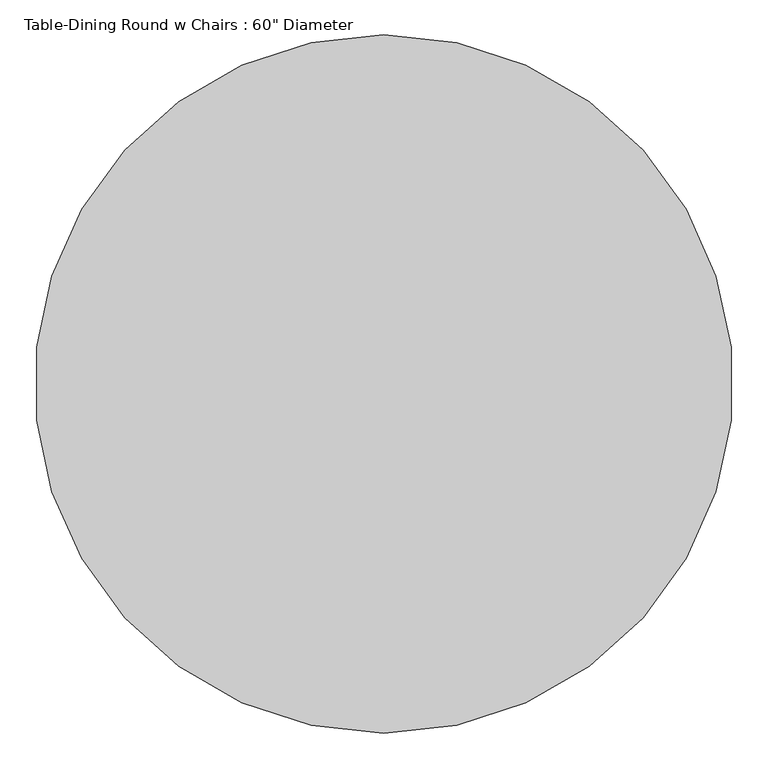
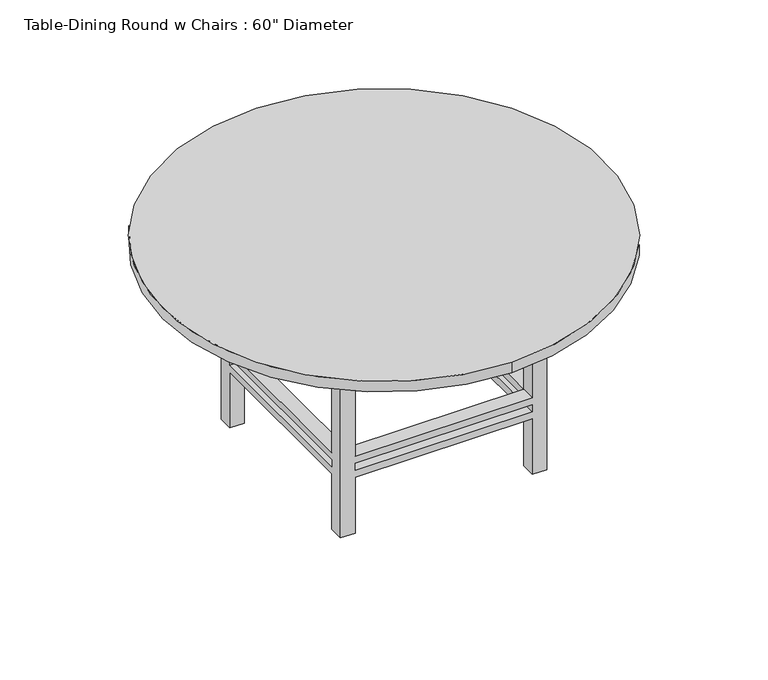
"""IFC4 building model written with IfcOpenShell, lengths in millimetres: furniture geometry."""

import ifcopenshell
import ifcopenshell.guid

model = None  # the IFC model being written
_history = None  # IfcOwnerHistory: only IFC2X3 demands one
_inside = {}  # id of a spatial element -> (the spatial element, [elements in it])
_under = {}  # id of a project, library or spatial element -> (it, [spatial elements below it])
_declared = {}  # id of a project -> (the project, [libraries it declares])
_typed = {}  # id of a type object -> (the type object, [elements of that type])
_made_of = {}  # id of a material, layer set ... -> (it, [elements and type objects made of it])


def new_model(schema):
    """Start an empty IFC model of exactly this schema.

    Asked for "IFC4X3", IfcOpenShell would pick the latest addendum, in which some entities
    have other attributes; the version numbers below select the first issue.
    IFC2X3 requires an IfcOwnerHistory on every rooted entity: one is made here for all.
    """
    global model, _history
    if schema == "IFC4X3":
        model = ifcopenshell.file(schema_version=(4, 3, 0, 0))
    else:
        model = ifcopenshell.file(schema=schema)
    _inside.clear()
    _under.clear()
    _declared.clear()
    _typed.clear()
    _made_of.clear()
    _history = None
    if model.schema == "IFC2X3":
        org = make("IfcOrganization", Name="unknown")
        user = make(
            "IfcPersonAndOrganization",
            ThePerson=make("IfcPerson", FamilyName="unknown"),
            TheOrganization=org,
        )
        app = make(
            "IfcApplication",
            ApplicationDeveloper=org,
            Version="unknown",
            ApplicationFullName="unknown",
            ApplicationIdentifier="unknown",
        )
        _history = make(
            "IfcOwnerHistory",
            OwningUser=user,
            OwningApplication=app,
            ChangeAction="ADDED",
            CreationDate=0,
        )
    return model


def make(cls, **values):
    """One entity of the class cls with the attributes given. An attribute that is None is left unset."""
    return model.create_entity(
        cls, **{name: value for name, value in values.items() if value is not None}
    )


def rooted(cls, **values):
    """An entity with a GlobalId (a new one), such as an element, a storey or a relation."""
    return make(cls, GlobalId=ifcopenshell.guid.new(), OwnerHistory=_history, **values)


def si_unit(unit_type, name, prefix=None):
    """IfcSIUnit, for example si_unit("LENGTHUNIT", "METRE", prefix="MILLI")."""
    return make("IfcSIUnit", UnitType=unit_type, Prefix=prefix, Name=name)


def assignment(units):
    """IfcUnitAssignment: the units of a project."""
    return None if units is None else make("IfcUnitAssignment", Units=units)


def point(xyz):
    """IfcCartesianPoint."""
    return None if xyz is None else make("IfcCartesianPoint", Coordinates=xyz)


def direction(xyz):
    """IfcDirection."""
    return None if xyz is None else make("IfcDirection", DirectionRatios=xyz)


def frame(location, z_axis=None, x_axis=None):
    """IfcAxis2Placement3D, a coordinate frame: its origin and axes. An axis left out is left unset."""
    return make(
        "IfcAxis2Placement3D",
        Location=point(location),
        Axis=direction(z_axis),
        RefDirection=direction(x_axis),
    )


def frame_2d(location, x_axis=None):
    """IfcAxis2Placement2D, a coordinate frame in the plane: its origin and x axis."""
    return make(
        "IfcAxis2Placement2D", Location=point(location), RefDirection=direction(x_axis)
    )


def origin():
    """The frame at (0, 0, 0) with its axes left unset."""
    return frame((0.0, 0.0, 0.0))


def place(relative_to, where):
    """IfcLocalPlacement: puts the frame where relative to a parent placement (None: the world)."""
    return make(
        "IfcLocalPlacement", PlacementRelTo=relative_to, RelativePlacement=where
    )


def context(
    kind, dimensions, precision=None, world=None, true_north=None, identifier=None
):
    """IfcGeometricRepresentationContext, for example the 3D "Model" context."""
    return make(
        "IfcGeometricRepresentationContext",
        ContextIdentifier=identifier,
        ContextType=kind,
        CoordinateSpaceDimension=dimensions,
        Precision=precision,
        WorldCoordinateSystem=world,
        TrueNorth=true_north,
    )


def project(units=None, contexts=None):
    """IfcProject with its units and contexts."""
    return rooted(
        "IfcProject",
        Name="project",
        RepresentationContexts=contexts,
        UnitsInContext=assignment(units),
    )


def spatial(cls, under=None, at=None, **own):
    """A site, building, storey or space (cls), placed at a placement, below another one or the project."""
    s = rooted(cls, ObjectPlacement=at, **own)
    if under is not None:
        _under.setdefault(under.id(), (under, []))[1].append(s)
    return s


def polyline(points):
    """IfcPolyline through the points."""
    return make("IfcPolyline", Points=[point(p) for p in points])


def circle_curve(where, radius):
    """IfcCircle in the frame where."""
    return make("IfcCircle", Position=where, Radius=radius)


def trimmed(basis, trim1, trim2, sense, master):
    """IfcTrimmedCurve: the piece of a basis curve between two trims."""
    return make(
        "IfcTrimmedCurve",
        BasisCurve=basis,
        Trim1=trim1,
        Trim2=trim2,
        SenseAgreement=sense,
        MasterRepresentation=master,
    )


def segment(curve, same_sense, transition):
    """IfcCompositeCurveSegment."""
    return make(
        "IfcCompositeCurveSegment",
        Transition=transition,
        SameSense=same_sense,
        ParentCurve=curve,
    )


def composite_curve(segments, self_intersect=None):
    """IfcCompositeCurve: segments joined end to end."""
    return make("IfcCompositeCurve", Segments=segments, SelfIntersect=self_intersect)


def outline(outer, holes=None, kind="AREA"):
    """IfcArbitraryClosedProfileDef: a profile drawn as a closed curve; with holes, ...WithVoids."""
    if holes is None:
        return make("IfcArbitraryClosedProfileDef", ProfileType=kind, OuterCurve=outer)
    return make(
        "IfcArbitraryProfileDefWithVoids",
        ProfileType=kind,
        OuterCurve=outer,
        InnerCurves=holes,
    )


def extrude(swept, where, along, depth):
    """IfcExtrudedAreaSolid: the profile swept, set in the frame where, extruded along a direction by depth."""
    return make(
        "IfcExtrudedAreaSolid",
        SweptArea=swept,
        Position=where,
        ExtrudedDirection=direction(along),
        Depth=depth,
    )


def faces_of(points, faces, orient=None, outer=None):
    """IfcFace entities. A face is a list of loops; a loop is a list of indices into points, from 0.

    orient and outer hold one flag for each loop. By default every Orientation is true, the
    first loop of a face is its IfcFaceOuterBound and the others are IfcFaceBound.
    """
    made = []
    for i, loops in enumerate(faces):
        bounds = []
        for j, loop in enumerate(loops):
            is_outer = j == 0 if outer is None else outer[i][j]
            bounds.append(
                make(
                    "IfcFaceOuterBound" if is_outer else "IfcFaceBound",
                    Bound=make("IfcPolyLoop", Polygon=[points[k] for k in loop]),
                    Orientation=True if orient is None else orient[i][j],
                )
            )
        made.append(make("IfcFace", Bounds=bounds))
    return made


def faceted_brep(points, faces, orient=None, outer=None, voids=None):
    """IfcFacetedBrep: a solid bounded by flat faces; with voids (closed shells), ...WithVoids."""
    shared = [point(p) for p in points]
    hull = make("IfcClosedShell", CfsFaces=faces_of(shared, faces, orient, outer))
    if voids is None:
        return make("IfcFacetedBrep", Outer=hull)
    return make(
        "IfcFacetedBrepWithVoids",
        Outer=hull,
        Voids=[
            make(cls, CfsFaces=faces_of(shared, fs, o, b)) for cls, fs, o, b in voids
        ],
    )


def shape(context_of_items, identifier, shape_type, items):
    """IfcShapeRepresentation: the items that make up one representation, for example the "Body"."""
    return make(
        "IfcShapeRepresentation",
        ContextOfItems=context_of_items,
        RepresentationIdentifier=identifier,
        RepresentationType=shape_type,
        Items=items,
    )


def source(mapping_origin, context_of_items, identifier, shape_type, items):
    """IfcRepresentationMap: a shape defined once, which mapped items show again and again."""
    return make(
        "IfcRepresentationMap",
        MappingOrigin=mapping_origin,
        MappedRepresentation=shape(context_of_items, identifier, shape_type, items),
    )


def transform(
    local_origin,
    x_axis=None,
    y_axis=None,
    z_axis=None,
    scale=None,
    scale2=None,
    scale3=None,
    uniform=True,
):
    """IfcCartesianTransformationOperator3D, or its non-uniform kind. x_axis, y_axis, z_axis: its Axis1, 2, 3."""
    if uniform:
        return make(
            "IfcCartesianTransformationOperator3D",
            Axis1=direction(x_axis),
            Axis2=direction(y_axis),
            LocalOrigin=point(local_origin),
            Scale=scale,
            Axis3=direction(z_axis),
        )
    return make(
        "IfcCartesianTransformationOperator3DnonUniform",
        Axis1=direction(x_axis),
        Axis2=direction(y_axis),
        LocalOrigin=point(local_origin),
        Scale=scale,
        Axis3=direction(z_axis),
        Scale2=scale2,
        Scale3=scale3,
    )


def mapped(mapping_source, mapping_target):
    """IfcMappedItem: shows the shape of a source again, moved by a transform."""
    return make(
        "IfcMappedItem", MappingSource=mapping_source, MappingTarget=mapping_target
    )


def made_of(thing, what):
    """Note that an element or type object is made of a material, layer set ...; save() writes the relation."""
    if what is not None:
        _made_of.setdefault(what.id(), (what, []))[1].append(thing)
    return thing


def element(
    cls,
    number,
    at=None,
    inside=None,
    cuts=None,
    type_object=None,
    material=None,
    context=None,
    identifier="Body",
    shape_type=None,
    held_by="IfcProductDefinitionShape",
    body=None,
    shapes=None,
    **own,
):
    """One element of the class cls, such as IfcWall. Its Tag is "e" and its number.

    at: its placement. inside: the storey or other place that contains it. cuts: it is an
    opening in that element (IfcRelVoidsElement). A single representation is given by context,
    identifier, shape_type and body (its items); several are given by shapes. held_by: the class
    of the entity that holds the representations. save() writes the other relations.
    """
    e = rooted(cls, Tag="e%d" % number, ObjectPlacement=at, **own)
    if body is not None:
        shapes = [shape(context, identifier, shape_type, body)]
    if shapes is not None:
        e.Representation = make(held_by, Representations=shapes)
    if inside is not None:
        _inside.setdefault(inside.id(), (inside, []))[1].append(e)
    if cuts is not None:
        rooted(
            "IfcRelVoidsElement", RelatingBuildingElement=cuts, RelatedOpeningElement=e
        )
    if type_object is not None:
        _typed.setdefault(type_object.id(), (type_object, []))[1].append(e)
    return made_of(e, material)


def aggregate(whole, parts):
    """IfcRelAggregates: a whole, such as a stair, and the parts it consists of."""
    return rooted("IfcRelAggregates", RelatingObject=whole, RelatedObjects=parts)


def save(model, path):
    """Write the relations noted so far, then the file.

    IfcRelAggregates (storeys below a building ...), IfcRelContainedInSpatialStructure (elements
    in a storey), IfcRelDefinesByType, IfcRelAssociatesMaterial and IfcRelDeclares: one each for
    every whole, place, type object, material and project.
    """
    for whole, parts in _under.values():
        aggregate(whole, parts)
    for where, things in _inside.values():
        rooted(
            "IfcRelContainedInSpatialStructure",
            RelatedElements=things,
            RelatingStructure=where,
        )
    for kind, things in _typed.values():
        rooted("IfcRelDefinesByType", RelatedObjects=things, RelatingType=kind)
    for what, things in _made_of.values():
        rooted("IfcRelAssociatesMaterial", RelatedObjects=things, RelatingMaterial=what)
    for by, libraries in _declared.values():
        rooted("IfcRelDeclares", RelatingContext=by, RelatedDefinitions=libraries)
    model.write(path)


def furniture_bbcc68ce(model_context):
    return source(origin(), model_context, "Body", "SolidModel", [
        faceted_brep([(408.4819672, 119.9213115, 279.4), (408.4819672, -489.6786885, 279.4), (459.2819672, -489.6786885, 279.4), (459.2819672, 119.9213115, 279.4), (-201.1180328, -489.6786885, 279.4), (-201.1180328, -540.4786885, 279.4), (408.4819672, -540.4786885, 279.4), (-201.1180328, 119.9213115, 279.4), (-251.9180328, 119.9213115, 279.4), (-251.9180328, -489.6786885, 279.4), (408.4819672, 170.7213115, 279.4), (-201.1180328, 170.7213115, 279.4), (408.4819672, 119.9213115, 254.0), (-201.1180328, 119.9213115, 254.0), (-201.1180328, 170.7213115, 254.0), (408.4819672, 170.7213115, 254.0), (-201.1180328, -489.6786885, 254.0), (-251.9180328, -489.6786885, 254.0), (-251.9180328, 119.9213115, 254.0), (408.4819672, -489.6786885, 254.0), (408.4819672, -540.4786885, 254.0), (-201.1180328, -540.4786885, 254.0), (459.2819672, 119.9213115, 254.0), (459.2819672, -489.6786885, 254.0), (-251.9180328, 170.7213115, 647.7), (-201.1180328, 170.7213115, 647.7), (408.4819672, 170.7213115, 647.7), (459.2819672, 170.7213115, 647.7), (459.2819672, 170.7213115, 0.0), (408.4819672, 170.7213115, 0.0), (408.4819672, 170.7213115, 203.2), (-201.1180328, 170.7213115, 203.2), (-201.1180328, 170.7213115, 0.0), (-251.9180328, 170.7213115, 0.0), (-201.1180328, 170.7213115, 228.6), (408.4819672, 170.7213115, 228.6), (-251.9180328, 119.9213115, 647.7), (-251.9180328, 119.9213115, 0.0), (-251.9180328, 119.9213115, 203.2), (-251.9180328, -489.6786885, 203.2), (-251.9180328, -489.6786885, 0.0), (-251.9180328, -540.4786885, 0.0), (-251.9180328, -540.4786885, 647.7), (-251.9180328, -489.6786885, 647.7), (-251.9180328, -489.6786885, 228.6), (-251.9180328, 119.9213115, 228.6), (459.2819672, -540.4786885, 647.7), (408.4819672, -540.4786885, 647.7), (-201.1180328, -540.4786885, 647.7), (-201.1180328, -540.4786885, 0.0), (-201.1180328, -540.4786885, 203.2), (408.4819672, -540.4786885, 203.2), (408.4819672, -540.4786885, 0.0), (459.2819672, -540.4786885, 0.0), (408.4819672, -540.4786885, 228.6), (-201.1180328, -540.4786885, 228.6), (459.2819672, 119.9213115, 647.7), (459.2819672, -489.6786885, 647.7), (459.2819672, -489.6786885, 0.0), (459.2819672, -489.6786885, 203.2), (459.2819672, 119.9213115, 203.2), (459.2819672, 119.9213115, 0.0), (459.2819672, 119.9213115, 228.6), (459.2819672, -489.6786885, 228.6), (-201.1180328, 119.9213115, 647.7), (408.4819672, -489.6786885, 647.7), (408.4819672, 119.9213115, 647.7), (-201.1180328, -489.6786885, 647.7), (408.4819672, 119.9213115, 0.0), (-201.1180328, -489.6786885, 0.0), (-201.1180328, 119.9213115, 0.0), (408.4819672, -489.6786885, 0.0), (-201.1180328, 119.9213115, 228.6), (-201.1180328, 119.9213115, 203.2), (408.4819672, 119.9213115, 228.6), (408.4819672, 119.9213115, 203.2), (408.4819672, -489.6786885, 228.6), (408.4819672, -489.6786885, 203.2), (-201.1180328, -489.6786885, 228.6), (-201.1180328, -489.6786885, 203.2)], [[[0, 1, 2, 3]], [[1, 4, 5, 6]], [[4, 7, 8, 9]], [[7, 0, 10, 11]], [[12, 13, 14, 15]], [[13, 16, 17, 18]], [[16, 19, 20, 21]], [[19, 12, 22, 23]], [[24, 25, 11, 10, 26, 27, 28, 29, 30, 31, 32, 33], [14, 34, 35, 15]], [[36, 24, 33, 37, 38, 39, 40, 41, 42, 43, 9, 8], [17, 44, 45, 18]], [[46, 47, 6, 5, 48, 42, 41, 49, 50, 51, 52, 53], [20, 54, 55, 21]], [[28, 27, 56, 3, 2, 57, 46, 53, 58, 59, 60, 61], [22, 62, 63, 23]], [[1, 0, 12, 19]], [[4, 1, 19, 16]], [[7, 4, 16, 13]], [[0, 7, 13, 12]], [[25, 24, 36, 64]], [[47, 46, 57, 65]], [[26, 66, 56, 27]], [[48, 67, 43, 42]], [[29, 28, 61, 68]], [[49, 41, 40, 69]], [[32, 70, 37, 33]], [[52, 71, 58, 53]], [[13, 18, 45, 72]], [[64, 36, 8, 7]], [[37, 70, 73, 38]], [[14, 13, 72, 34]], [[25, 64, 7, 11]], [[70, 32, 31, 73]], [[12, 15, 35, 74]], [[66, 26, 10, 0]], [[29, 68, 75, 30]], [[22, 12, 74, 62]], [[56, 66, 0, 3]], [[68, 61, 60, 75]], [[19, 23, 63, 76]], [[65, 57, 2, 1]], [[58, 71, 77, 59]], [[20, 19, 76, 54]], [[47, 65, 1, 6]], [[71, 52, 51, 77]], [[16, 21, 55, 78]], [[67, 48, 5, 4]], [[49, 69, 79, 50]], [[17, 16, 78, 44]], [[43, 67, 4, 9]], [[69, 40, 39, 79]], [[74, 76, 63, 62]], [[76, 78, 55, 54]], [[78, 72, 45, 44]], [[72, 74, 35, 34]], [[75, 73, 31, 30]], [[73, 79, 39, 38]], [[79, 77, 51, 50]], [[77, 75, 60, 59]], [[76, 74, 75, 77]], [[78, 76, 77, 79]], [[72, 78, 79, 73]], [[74, 72, 73, 75]]]),
        extrude(outline(polyline([(484.6819672, 196.1213115), (484.6819672, -565.8786885), (-277.3180328, -565.8786885), (-277.3180328, 196.1213115), (484.6819672, 196.1213115)]), holes=[polyline([(459.2819672, 170.7213115), (-251.9180328, 170.7213115), (-251.9180328, -540.4786885), (459.2819672, -540.4786885), (459.2819672, 170.7213115)])]), frame((0.0, 0.0, 647.7), z_axis=(0.0, 0.0, 1.0), x_axis=(1.0, 0.0, 0.0)), (0.0, 0.0, 1.0), 76.2),
        extrude(outline(composite_curve([segment(trimmed(circle_curve(frame_2d((103.6819672, -184.8786885)), 762.0), [point((103.6819672, -946.8786885))], [point((103.6819672, 577.1213115))], False, "CARTESIAN"), True, "CONTINUOUS"), segment(trimmed(circle_curve(frame_2d((103.6819672, -184.8786885)), 762.0), [point((103.6819672, 577.1213115))], [point((103.6819672, -946.8786885))], False, "CARTESIAN"), True, "CONTINUOUS")], self_intersect=False)), frame((0.0, 0.0, 723.9), z_axis=(0.0, 0.0, 1.0), x_axis=(1.0, 0.0, 0.0)), (0.0, 0.0, 1.0), 38.1),
    ])


if __name__ == "__main__":
    model = new_model("IFC4")
    model_context = context("Model", 3, world=origin())
    ifc_project = project(units=[si_unit("LENGTHUNIT", "METRE", prefix="MILLI")], contexts=[model_context])
    site = spatial("IfcSite", under=ifc_project)
    building = spatial("IfcBuilding", under=site)
    placement = place(None, origin())
    furniture_shape = furniture_bbcc68ce(model_context)
    element("IfcFurniture", 1, ObjectType="Table-Dining Round w Chairs : 60\" Diameter", at=placement, inside=building, context=model_context, shape_type="MappedRepresentation", body=[
        mapped(furniture_shape, transform((0.0, 0.0, 0.0), x_axis=(1.0, 0.0, 0.0), y_axis=(0.0, 1.0, 0.0), z_axis=(0.0, 0.0, 1.0))),
    ])
    save(model, "model.ifc")

# Revit data of these elements
# Type "Table-Dining Round w Chairs : 60\" Diameter"
#   Assembly Code = "E2020200"
#   Radius = 2' - 6"
#   Diameter = 5' - 0"
#   Height = 2' - 6"
#   Chairs = 6
#   Base Material = Pine
#   Top Material = Laminate, Linen, Matte
# Element 1 (IfcFurniture, "Table-Dining Round w Chairs : 60\" Diameter")
#   Materials on its faces: "Pine", "Laminate, Linen, Matte"
# Materials
#   "Pine": class "Wood", colour RGB 223 192 134, transparency 0, Description = "Pinus Echinata", Cost = 0
#   "Laminate, Linen, Matte": class "Plastic", colour RGB 249 239 230, transparency 0, Description = "Plastic Laminate - Linen, Matte", Cost = 0
